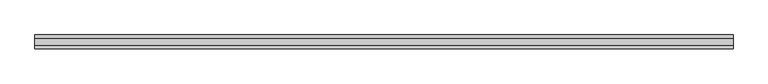
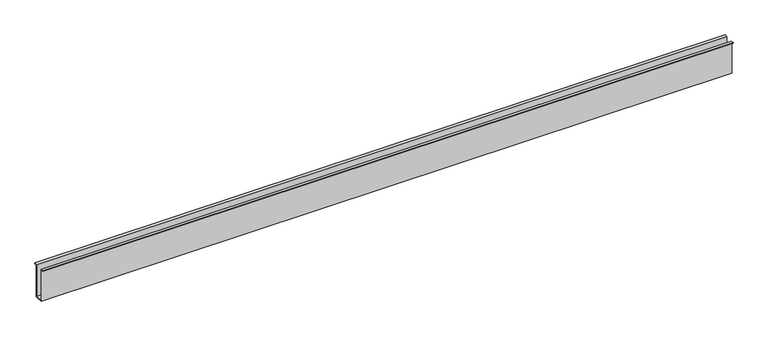
"""IFC4 building model written with IfcOpenShell, lengths in millimetres: railing geometry, ML_Perfil U de embutir2 : ML_Perfil U de embutir."""

import ifcopenshell
import ifcopenshell.guid

model = None  # the IFC model being written
_history = None  # IfcOwnerHistory: only IFC2X3 demands one
_inside = {}  # id of a spatial element -> (the spatial element, [elements in it])
_under = {}  # id of a project, library or spatial element -> (it, [spatial elements below it])
_declared = {}  # id of a project -> (the project, [libraries it declares])
_typed = {}  # id of a type object -> (the type object, [elements of that type])
_made_of = {}  # id of a material, layer set ... -> (it, [elements and type objects made of it])


def new_model(schema):
    """Start an empty IFC model of exactly this schema.

    Asked for "IFC4X3", IfcOpenShell would pick the latest addendum, in which some entities
    have other attributes; the version numbers below select the first issue.
    IFC2X3 requires an IfcOwnerHistory on every rooted entity: one is made here for all.
    """
    global model, _history
    if schema == "IFC4X3":
        model = ifcopenshell.file(schema_version=(4, 3, 0, 0))
    else:
        model = ifcopenshell.file(schema=schema)
    _inside.clear()
    _under.clear()
    _declared.clear()
    _typed.clear()
    _made_of.clear()
    _history = None
    if model.schema == "IFC2X3":
        org = make("IfcOrganization", Name="unknown")
        user = make(
            "IfcPersonAndOrganization",
            ThePerson=make("IfcPerson", FamilyName="unknown"),
            TheOrganization=org,
        )
        app = make(
            "IfcApplication",
            ApplicationDeveloper=org,
            Version="unknown",
            ApplicationFullName="unknown",
            ApplicationIdentifier="unknown",
        )
        _history = make(
            "IfcOwnerHistory",
            OwningUser=user,
            OwningApplication=app,
            ChangeAction="ADDED",
            CreationDate=0,
        )
    return model


def make(cls, **values):
    """One entity of the class cls with the attributes given. An attribute that is None is left unset."""
    return model.create_entity(
        cls, **{name: value for name, value in values.items() if value is not None}
    )


def rooted(cls, **values):
    """An entity with a GlobalId (a new one), such as an element, a storey or a relation."""
    return make(cls, GlobalId=ifcopenshell.guid.new(), OwnerHistory=_history, **values)


def si_unit(unit_type, name, prefix=None):
    """IfcSIUnit, for example si_unit("LENGTHUNIT", "METRE", prefix="MILLI")."""
    return make("IfcSIUnit", UnitType=unit_type, Prefix=prefix, Name=name)


def assignment(units):
    """IfcUnitAssignment: the units of a project."""
    return None if units is None else make("IfcUnitAssignment", Units=units)


def point(xyz):
    """IfcCartesianPoint."""
    return None if xyz is None else make("IfcCartesianPoint", Coordinates=xyz)


def direction(xyz):
    """IfcDirection."""
    return None if xyz is None else make("IfcDirection", DirectionRatios=xyz)


def frame(location, z_axis=None, x_axis=None):
    """IfcAxis2Placement3D, a coordinate frame: its origin and axes. An axis left out is left unset."""
    return make(
        "IfcAxis2Placement3D",
        Location=point(location),
        Axis=direction(z_axis),
        RefDirection=direction(x_axis),
    )


def origin():
    """The frame at (0, 0, 0) with its axes left unset."""
    return frame((0.0, 0.0, 0.0))


def place(relative_to, where):
    """IfcLocalPlacement: puts the frame where relative to a parent placement (None: the world)."""
    return make(
        "IfcLocalPlacement", PlacementRelTo=relative_to, RelativePlacement=where
    )


def context(
    kind, dimensions, precision=None, world=None, true_north=None, identifier=None
):
    """IfcGeometricRepresentationContext, for example the 3D "Model" context."""
    return make(
        "IfcGeometricRepresentationContext",
        ContextIdentifier=identifier,
        ContextType=kind,
        CoordinateSpaceDimension=dimensions,
        Precision=precision,
        WorldCoordinateSystem=world,
        TrueNorth=true_north,
    )


def project(units=None, contexts=None):
    """IfcProject with its units and contexts."""
    return rooted(
        "IfcProject",
        Name="project",
        RepresentationContexts=contexts,
        UnitsInContext=assignment(units),
    )


def spatial(cls, under=None, at=None, **own):
    """A site, building, storey or space (cls), placed at a placement, below another one or the project."""
    s = rooted(cls, ObjectPlacement=at, **own)
    if under is not None:
        _under.setdefault(under.id(), (under, []))[1].append(s)
    return s


def polyline(points):
    """IfcPolyline through the points."""
    return make("IfcPolyline", Points=[point(p) for p in points])


def outline(outer, holes=None, kind="AREA"):
    """IfcArbitraryClosedProfileDef: a profile drawn as a closed curve; with holes, ...WithVoids."""
    if holes is None:
        return make("IfcArbitraryClosedProfileDef", ProfileType=kind, OuterCurve=outer)
    return make(
        "IfcArbitraryProfileDefWithVoids",
        ProfileType=kind,
        OuterCurve=outer,
        InnerCurves=holes,
    )


def extrude(swept, where, along, depth):
    """IfcExtrudedAreaSolid: the profile swept, set in the frame where, extruded along a direction by depth."""
    return make(
        "IfcExtrudedAreaSolid",
        SweptArea=swept,
        Position=where,
        ExtrudedDirection=direction(along),
        Depth=depth,
    )


def shape(context_of_items, identifier, shape_type, items):
    """IfcShapeRepresentation: the items that make up one representation, for example the "Body"."""
    return make(
        "IfcShapeRepresentation",
        ContextOfItems=context_of_items,
        RepresentationIdentifier=identifier,
        RepresentationType=shape_type,
        Items=items,
    )


def source(mapping_origin, context_of_items, identifier, shape_type, items):
    """IfcRepresentationMap: a shape defined once, which mapped items show again and again."""
    return make(
        "IfcRepresentationMap",
        MappingOrigin=mapping_origin,
        MappedRepresentation=shape(context_of_items, identifier, shape_type, items),
    )


def transform(
    local_origin,
    x_axis=None,
    y_axis=None,
    z_axis=None,
    scale=None,
    scale2=None,
    scale3=None,
    uniform=True,
):
    """IfcCartesianTransformationOperator3D, or its non-uniform kind. x_axis, y_axis, z_axis: its Axis1, 2, 3."""
    if uniform:
        return make(
            "IfcCartesianTransformationOperator3D",
            Axis1=direction(x_axis),
            Axis2=direction(y_axis),
            LocalOrigin=point(local_origin),
            Scale=scale,
            Axis3=direction(z_axis),
        )
    return make(
        "IfcCartesianTransformationOperator3DnonUniform",
        Axis1=direction(x_axis),
        Axis2=direction(y_axis),
        LocalOrigin=point(local_origin),
        Scale=scale,
        Axis3=direction(z_axis),
        Scale2=scale2,
        Scale3=scale3,
    )


def mapped(mapping_source, mapping_target):
    """IfcMappedItem: shows the shape of a source again, moved by a transform."""
    return make(
        "IfcMappedItem", MappingSource=mapping_source, MappingTarget=mapping_target
    )


def made_of(thing, what):
    """Note that an element or type object is made of a material, layer set ...; save() writes the relation."""
    if what is not None:
        _made_of.setdefault(what.id(), (what, []))[1].append(thing)
    return thing


def element(
    cls,
    number,
    at=None,
    inside=None,
    cuts=None,
    type_object=None,
    material=None,
    context=None,
    identifier="Body",
    shape_type=None,
    held_by="IfcProductDefinitionShape",
    body=None,
    shapes=None,
    **own,
):
    """One element of the class cls, such as IfcWall. Its Tag is "e" and its number.

    at: its placement. inside: the storey or other place that contains it. cuts: it is an
    opening in that element (IfcRelVoidsElement). A single representation is given by context,
    identifier, shape_type and body (its items); several are given by shapes. held_by: the class
    of the entity that holds the representations. save() writes the other relations.
    """
    e = rooted(cls, Tag="e%d" % number, ObjectPlacement=at, **own)
    if body is not None:
        shapes = [shape(context, identifier, shape_type, body)]
    if shapes is not None:
        e.Representation = make(held_by, Representations=shapes)
    if inside is not None:
        _inside.setdefault(inside.id(), (inside, []))[1].append(e)
    if cuts is not None:
        rooted(
            "IfcRelVoidsElement", RelatingBuildingElement=cuts, RelatedOpeningElement=e
        )
    if type_object is not None:
        _typed.setdefault(type_object.id(), (type_object, []))[1].append(e)
    return made_of(e, material)


def aggregate(whole, parts):
    """IfcRelAggregates: a whole, such as a stair, and the parts it consists of."""
    return rooted("IfcRelAggregates", RelatingObject=whole, RelatedObjects=parts)


def save(model, path):
    """Write the relations noted so far, then the file.

    IfcRelAggregates (storeys below a building ...), IfcRelContainedInSpatialStructure (elements
    in a storey), IfcRelDefinesByType, IfcRelAssociatesMaterial and IfcRelDeclares: one each for
    every whole, place, type object, material and project.
    """
    for whole, parts in _under.values():
        aggregate(whole, parts)
    for where, things in _inside.values():
        rooted(
            "IfcRelContainedInSpatialStructure",
            RelatedElements=things,
            RelatingStructure=where,
        )
    for kind, things in _typed.values():
        rooted("IfcRelDefinesByType", RelatedObjects=things, RelatingType=kind)
    for what, things in _made_of.values():
        rooted("IfcRelAssociatesMaterial", RelatedObjects=things, RelatingMaterial=what)
    for by, libraries in _declared.values():
        rooted("IfcRelDeclares", RelatingContext=by, RelatedDefinitions=libraries)
    model.write(path)


def railing_c8eab29c(model_context):
    return source(origin(), model_context, "Body", "SweptSolid", [
        extrude(outline(polyline([(1832.4523952, 3702.0), (1832.4523952, 3594.0), (1856.4523952, 3594.0), (1856.4523952, 3702.0), (1866.9523952, 3702.0), (1866.9523952, 3700.0), (1858.4523952, 3700.0), (1858.4523952, 3592.0), (1830.4523952, 3592.0), (1830.4523952, 3700.0), (1821.9523952, 3700.0), (1821.9523952, 3702.0), (1832.4523952, 3702.0)])), frame((-12226.1487231, 0.0, 0.0), z_axis=(1.0, 0.0, 0.0), x_axis=(0.0, 1.0, 0.0)), (0.0, 0.0, 1.0), 2240.0),
    ])


if __name__ == "__main__":
    model = new_model("IFC4")
    model_context = context("Model", 3, world=origin())
    ifc_project = project(units=[si_unit("LENGTHUNIT", "METRE", prefix="MILLI")], contexts=[model_context])
    site = spatial("IfcSite", under=ifc_project)
    building = spatial("IfcBuilding", under=site)
    placement = place(None, origin())
    railing_shape = railing_c8eab29c(model_context)
    element("IfcRailing", 1, ObjectType="ML_Perfil U de embutir2 : ML_Perfil U de embutir", at=placement, inside=building, context=model_context, shape_type="MappedRepresentation", body=[
        mapped(railing_shape, transform((0.0, 0.0, 0.0), x_axis=(1.0, 0.0, 0.0), y_axis=(0.0, 1.0, 0.0), z_axis=(0.0, 0.0, 1.0))),
    ])
    save(model, "model.ifc")

# Revit data of these elements
# Type "ML_Perfil U de embutir2 : ML_Perfil U de embutir"
#   ME_Compr [instance default] = 2.24 m
#   ME_Material Perfil [instance default] = .ALUMÍNIO COM PINTURA ELETROSTÁTICA BRANCA
# Element 1 (IfcRailing, "ML_Perfil U de embutir2 : ML_Perfil U de embutir")
#   Materials on its faces: ".ALUMÍNIO COM PINTURA ELETROSTÁTICA BRANCA"
# Materials
#   ".ALUMÍNIO COM PINTURA ELETROSTÁTICA BRANCA": class "CC_METAIS", colour RGB 241 241 241, transparency 0, Cost = 0
